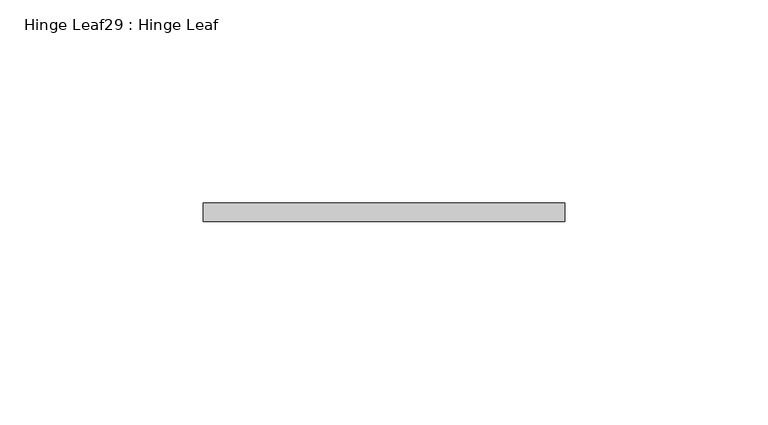
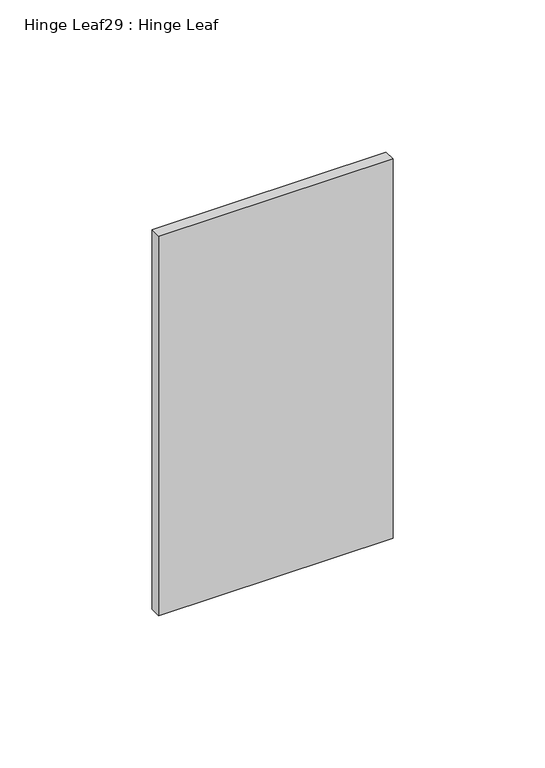
"""IFC4 building model written with IfcOpenShell, lengths in millimetres: proxy geometry, Hinge Leaf29 : Hinge Leaf."""

from ifc_helpers import new_model, si_unit, frame, origin, place, context, project, spatial, polyline, outline, extrude, source, transform, mapped, element, save


def hinge_leaf29_hinge_leaf_6d526917(model_context):
    return source(origin(), model_context, "Body", "SweptSolid", [
        extrude(outline(polyline([(587327.7934739, -531772.5663841), (587416.6934739, -531772.5663841), (587416.6934739, -531777.1383841), (587327.7934739, -531777.1383841), (587327.7934739, -531772.5663841)])), frame((0.0, 0.0, 1936.75), z_axis=(0.0, 0.0, 1.0), x_axis=(1.0, 0.0, 0.0)), (0.0, 0.0, 1.0), 152.4),
    ])


if __name__ == "__main__":
    model = new_model("IFC4")
    model_context = context("Model", 3, world=origin())
    ifc_project = project(units=[si_unit("LENGTHUNIT", "METRE", prefix="MILLI")], contexts=[model_context])
    site = spatial("IfcSite", under=ifc_project)
    building = spatial("IfcBuilding", under=site)
    placement = place(None, origin())
    hinge_leaf29_hinge_leaf_shape = hinge_leaf29_hinge_leaf_6d526917(model_context)
    element("IfcBuildingElementProxy", 1, Name="Hinge Leaf29 : Hinge Leaf", ObjectType="Hinge Leaf29 : Hinge Leaf", at=placement, inside=building, context=model_context, shape_type="MappedRepresentation", body=[
        mapped(hinge_leaf29_hinge_leaf_shape, transform((0.0, 0.0, 0.0), x_axis=(1.0, 0.0, 0.0), y_axis=(0.0, 1.0, 0.0), z_axis=(0.0, 0.0, 1.0))),
    ])
    save(model, "model.ifc")

# Revit data of these elements
# Element 1 (IfcBuildingElementProxy, "Hinge Leaf29 : Hinge Leaf")
#   Materials on its faces: "6\"X6\" WELD-ON STL BUTT HINGE"
# Materials
#   "6\"X6\" WELD-ON STL BUTT HINGE": class "Metal", colour RGB 189 187 185, transparency 0, Description = "Carbon steel", Cost = 0
